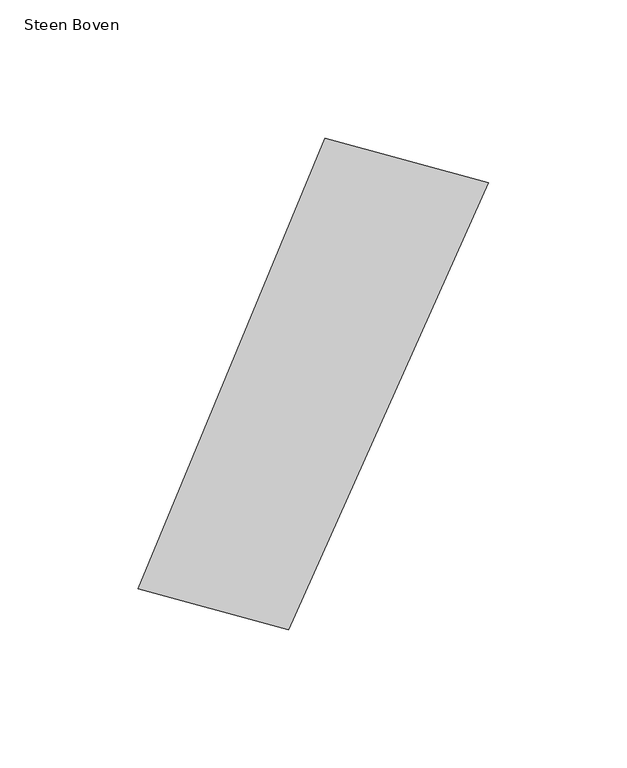
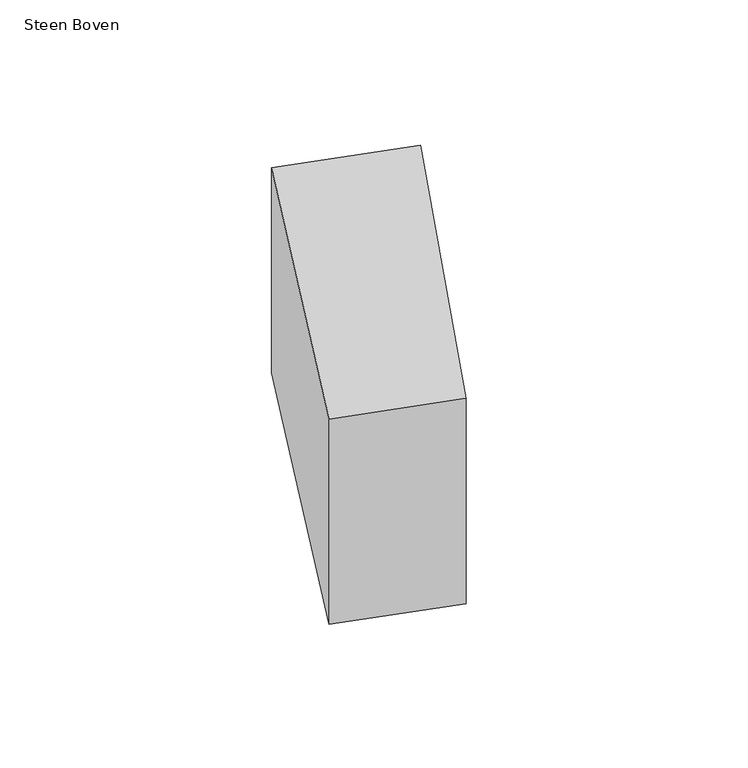
"""IFC4 building model written with IfcOpenShell, lengths in millimetres: proxy geometry, 00_GMA_steen_versie_4 : Steen Boven."""

from ifc_helpers import new_model, si_unit, origin, origin_with_axes, place, context, project, spatial, polyline, outline, extrude, source, transform, mapped, element, save


def steen_boven_db613410(model_context):
    return source(origin(), model_context, "Body", "SweptSolid", [
        extrude(outline(polyline([(137.9666665, 153.0531188), (65.533356, -8.6746975), (11.0862495, 6.1311783), (78.6858429, 169.1544645), (137.9666665, 153.0531188)])), origin_with_axes(), (0.0, 0.0, 1.0), 100.0),
    ])


if __name__ == "__main__":
    model = new_model("IFC4")
    model_context = context("Model", 3, world=origin())
    ifc_project = project(units=[si_unit("LENGTHUNIT", "METRE", prefix="MILLI")], contexts=[model_context])
    site = spatial("IfcSite", under=ifc_project)
    building = spatial("IfcBuilding", under=site)
    placement = place(None, origin())
    steen_boven_shape = steen_boven_db613410(model_context)
    element("IfcBuildingElementProxy", 1, Name="00_GMA_steen_versie_4 : Steen Boven", ObjectType="00_GMA_steen_versie_4 : Steen Boven", at=placement, inside=building, context=model_context, shape_type="MappedRepresentation", body=[
        mapped(steen_boven_shape, transform((0.0, 0.0, 0.0), x_axis=(1.0, 0.0, 0.0), y_axis=(0.0, 1.0, 0.0), z_axis=(0.0, 0.0, 1.0))),
    ])
    save(model, "model.ifc")

# Revit data of these elements
# Type "00_GMA_steen_versie_4 : Steen Boven"
#   StootVoegHalfBoven [instance default] = 5 mm
#   StootVoegHalf [instance default] = 5 mm
#   StootVoegBreedteOnder = 10 mm
#   StootVoegBreedteBoven = 10 mm
#   Steendikte = 100 mm
#   LintVoegOnderHalf = 5 mm
#   LintVoegOnder = 10 mm
#   LintVoegBovenHalf = 0 mm
#   LintVoegBoven = 0 mm
#   materiaal = none
#   MateriaalVoeg = none
#   Default Elevation = 0
